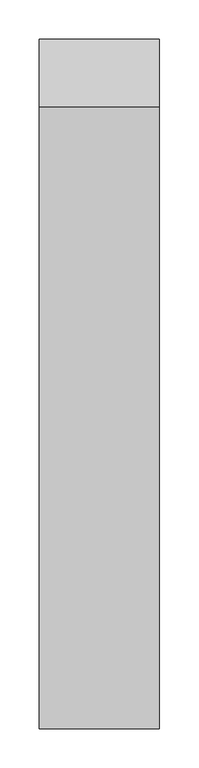
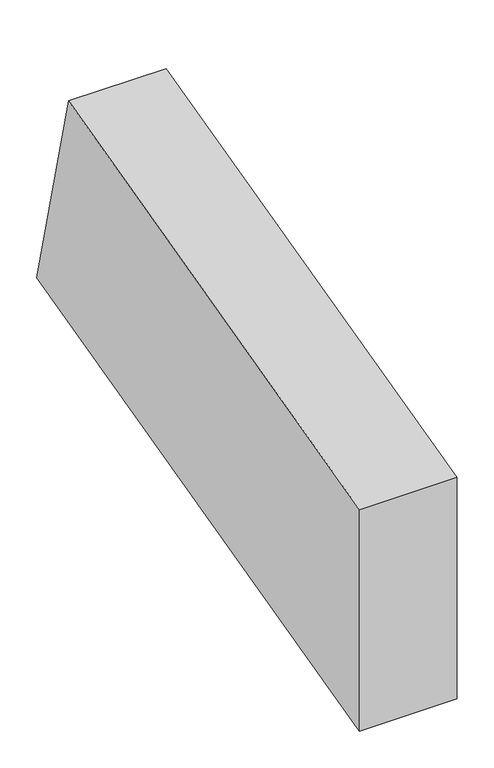
"""IFC4 building model written with IfcOpenShell, lengths in millimetres: proxy geometry, Framing017 3143 : Framing017 3143."""

from ifc_helpers import new_model, si_unit, frame, origin, place, context, project, spatial, polyline, outline, extrude, source, transform, mapped, element, save


def generic_models_1a04e2ea(model_context):
    return source(origin(), model_context, "Body", "SweptSolid", [
        extrude(outline(polyline([(8857.883325, 43384.4932401), (9647.0095123, 43581.9371332), (9733.2922309, 43237.0426118), (8857.883325, 43018.0404079), (8857.883325, 43384.4932401)])), frame((4322.6883192, 0.0, 0.0), z_axis=(1.0, 0.0, 0.0), x_axis=(0.0, 1.0, 0.0)), (0.0, 0.0, 1.0), 152.4),
    ])


if __name__ == "__main__":
    model = new_model("IFC4")
    model_context = context("Model", 3, world=origin())
    ifc_project = project(units=[si_unit("LENGTHUNIT", "METRE", prefix="MILLI")], contexts=[model_context])
    site = spatial("IfcSite", under=ifc_project)
    building = spatial("IfcBuilding", under=site)
    placement = place(None, origin())
    generic_models_shape = generic_models_1a04e2ea(model_context)
    element("IfcBuildingElementProxy", 1, Name="Framing017 3143 : Framing017 3143", ObjectType="Framing017 3143 : Framing017 3143", at=placement, inside=building, context=model_context, shape_type="MappedRepresentation", body=[
        mapped(generic_models_shape, transform((0.0, 0.0, 0.0), x_axis=(1.0, 0.0, 0.0), y_axis=(0.0, 1.0, 0.0), z_axis=(0.0, 0.0, 1.0))),
    ])
    save(model, "model.ifc")

# Revit data of these elements
# Type "Framing017 3143 : Framing017 3143"
#   NameOverride = "Framing017"
# Element 1 (IfcBuildingElementProxy, "Framing017 3143 : Framing017 3143")
#   Materials on its faces: "WOOD FRAMING (SEE STRUCT DWGS)"
# Materials
#   "WOOD FRAMING (SEE STRUCT DWGS)": class "Unassigned", colour RGB 224 188 168, transparency 0, Cost = 0
